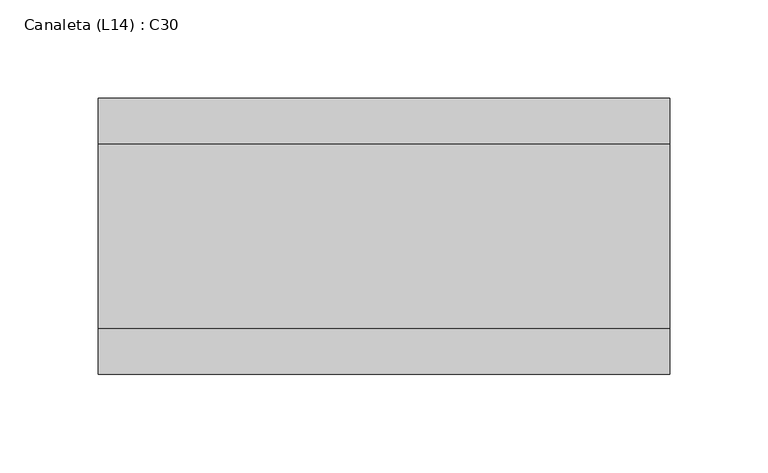
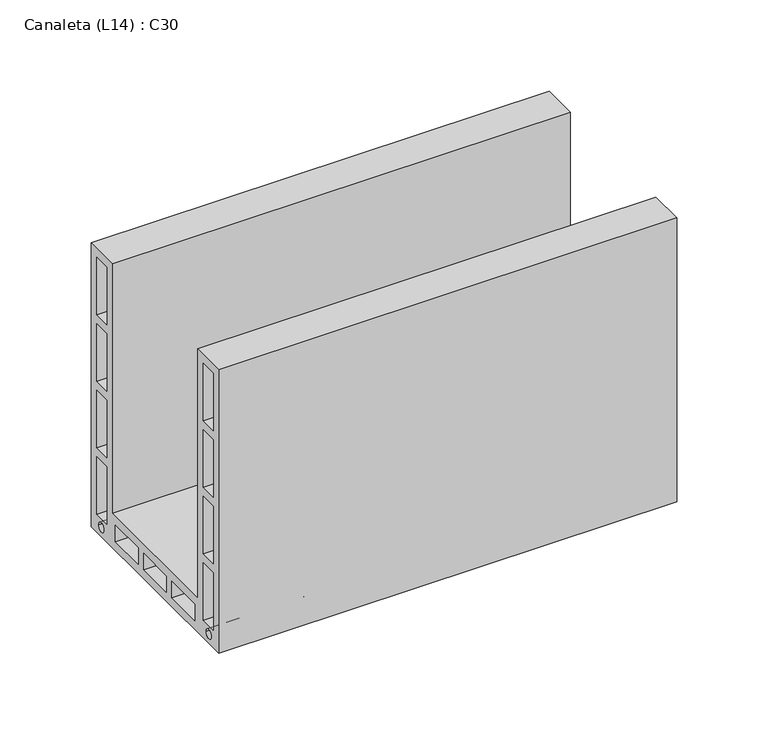
"""IFC4 building model written with IfcOpenShell, lengths in millimetres: proxy geometry, Canaleta (L14) : C30."""

from ifc_helpers import new_model, si_unit, point, frame, frame_2d, origin, place, context, project, spatial, polyline, circle_curve, trimmed, segment, composite_curve, outline, extrude, source, transform, mapped, element, save


def canaleta_l14_c30_6f9dc855(model_context):
    return source(origin(), model_context, "Body", "SweptSolid", [
        extrude(outline(polyline([(140.0, 0.0), (0.0, 0.0), (0.0, 190.0), (23.0, 190.0), (23.0, 23.0), (117.0, 23.0), (117.0, 190.0), (140.0, 190.0), (140.0, 0.0)]), holes=[polyline([(123.0, 184.0), (123.0, 145.5), (134.0, 145.5), (134.0, 184.0), (123.0, 184.0)]), polyline([(123.0, 139.5), (123.0, 101.0), (134.0, 101.0), (134.0, 139.5), (123.0, 139.5)]), polyline([(123.0, 95.0), (123.0, 56.5), (134.0, 56.5), (134.0, 95.0), (123.0, 95.0)]), polyline([(123.0, 50.5), (123.0, 12.0), (134.0, 12.0), (134.0, 50.5), (123.0, 50.5)]), composite_curve([segment(trimmed(circle_curve(frame_2d((128.9426557, 6.2112346)), 3.0), [point((125.9426557, 6.2112346))], [point((131.9426557, 6.2112346))], True, "CARTESIAN"), True, "CONTINUOUS"), segment(trimmed(circle_curve(frame_2d((128.9426557, 6.2112346)), 3.0), [point((131.9426557, 6.2112346))], [point((125.9426557, 6.2112346))], True, "CARTESIAN"), True, "CONTINUOUS")], self_intersect=False), polyline([(17.0, 184.0), (6.0, 184.0), (6.0, 145.5), (17.0, 145.5), (17.0, 184.0)]), polyline([(17.0, 139.5), (6.0, 139.5), (6.0, 101.0), (17.0, 101.0), (17.0, 139.5)]), polyline([(17.0, 95.0), (6.0, 95.0), (6.0, 56.5), (17.0, 56.5), (17.0, 95.0)]), polyline([(17.0, 50.5), (6.0, 50.5), (6.0, 12.0), (17.0, 12.0), (17.0, 50.5)]), composite_curve([segment(trimmed(circle_curve(frame_2d((11.0573443, 6.2112346)), 3.0), [point((8.0573443, 6.2112346))], [point((14.0573443, 6.2112346))], True, "CARTESIAN"), True, "CONTINUOUS"), segment(trimmed(circle_curve(frame_2d((11.0573443, 6.2112346)), 3.0), [point((14.0573443, 6.2112346))], [point((8.0573443, 6.2112346))], True, "CARTESIAN"), True, "CONTINUOUS")], self_intersect=False), polyline([(88.5, 17.0), (88.5, 6.0), (113.5, 6.0), (113.5, 17.0), (88.5, 17.0)]), polyline([(57.5, 17.0), (57.5, 6.0), (82.5, 6.0), (82.5, 17.0), (57.5, 17.0)]), polyline([(26.5, 17.0), (26.5, 6.0), (51.5, 6.0), (51.5, 17.0), (26.5, 17.0)])]), frame((0.0, 0.0, 0.0), z_axis=(1.0, 0.0, 0.0), x_axis=(0.0, 1.0, 0.0)), (0.0, 0.0, 1.0), 290.0),
    ])


if __name__ == "__main__":
    model = new_model("IFC4")
    model_context = context("Model", 3, world=origin())
    ifc_project = project(units=[si_unit("LENGTHUNIT", "METRE", prefix="MILLI")], contexts=[model_context])
    site = spatial("IfcSite", under=ifc_project)
    building = spatial("IfcBuilding", under=site)
    placement = place(None, origin())
    canaleta_l14_c30_shape = canaleta_l14_c30_6f9dc855(model_context)
    element("IfcBuildingElementProxy", 1, Name="Canaleta (L14) : C30", ObjectType="Canaleta (L14) : C30", at=placement, inside=building, context=model_context, shape_type="MappedRepresentation", body=[
        mapped(canaleta_l14_c30_shape, transform((0.0, 0.0, 0.0), x_axis=(1.0, 0.0, 0.0), y_axis=(0.0, 1.0, 0.0), z_axis=(0.0, 0.0, 1.0))),
    ])
    save(model, "model.ifc")

# Revit data of these elements
# Type "Canaleta (L14) : C30"
#   Comprimento = 0.290 m
#   Material [instance default] = Blocos Cerâmicos
#   Default Elevation = 0
# Element 1 (IfcBuildingElementProxy, "Canaleta (L14) : C30")
#   Materials on its faces: "Blocos Cerâmicos"
# Materials
#   "Blocos Cerâmicos": class "Genérico", colour RGB 177 84 47, transparency 0, Cost = 0
